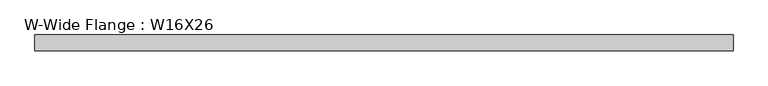
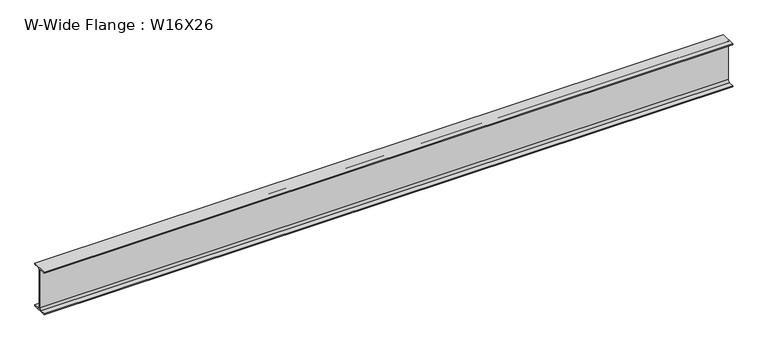
"""IFC4 building model written with IfcOpenShell, lengths in millimetres: beam geometry, W-Wide Flange : W16X26."""

from ifc_helpers import new_model, si_unit, point, frame, frame_2d, origin, place, context, project, spatial, polyline, circle_curve, trimmed, segment, composite_curve, outline, extrude, source, transform, mapped, element, save


def w_wide_flange_w16x26_1833ff5e(model_context):
    return source(origin(), model_context, "Body", "SweptSolid", [
        extrude(outline(composite_curve([segment(polyline([(69.85, -190.627), (69.85, -199.39), (-69.85, -199.39), (-69.85, -190.627), (-21.3995, -190.627)]), True, "CONTINUOUS"), segment(trimmed(circle_curve(frame_2d((-21.3995, -172.4025)), 18.2245), [point((-21.3995, -190.627))], [point((-3.175, -172.4025))], True, "CARTESIAN"), True, "CONTINUOUS"), segment(polyline([(-3.175, -172.4025), (-3.175, 172.4025)]), True, "CONTINUOUS"), segment(trimmed(circle_curve(frame_2d((-21.3995, 172.4025)), 18.2245), [point((-3.175, 172.4025))], [point((-21.3995, 190.627))], True, "CARTESIAN"), True, "CONTINUOUS"), segment(polyline([(-21.3995, 190.627), (-69.85, 190.627), (-69.85, 199.39), (69.85, 199.39), (69.85, 190.627), (21.3995, 190.627)]), True, "CONTINUOUS"), segment(trimmed(circle_curve(frame_2d((21.3995, 172.4025)), 18.2245), [point((21.3995, 190.627))], [point((3.175, 172.4025))], True, "CARTESIAN"), True, "CONTINUOUS"), segment(polyline([(3.175, 172.4025), (3.175, -172.4025)]), True, "CONTINUOUS"), segment(trimmed(circle_curve(frame_2d((21.3995, -172.4025)), 18.2245), [point((3.175, -172.4025))], [point((21.3995, -190.627))], True, "CARTESIAN"), True, "CONTINUOUS"), segment(polyline([(21.3995, -190.627), (69.85, -190.627)]), True, "CONTINUOUS")], self_intersect=False)), frame((-3048.0, 0.0, 0.0), z_axis=(1.0, 0.0, 0.0), x_axis=(0.0, 1.0, 0.0)), (0.0, 0.0, 1.0), 6096.0),
    ])


if __name__ == "__main__":
    model = new_model("IFC4")
    model_context = context("Model", 3, world=origin())
    ifc_project = project(units=[si_unit("LENGTHUNIT", "METRE", prefix="MILLI")], contexts=[model_context])
    site = spatial("IfcSite", under=ifc_project)
    building = spatial("IfcBuilding", under=site)
    placement = place(None, origin())
    w_wide_flange_w16x26_shape = w_wide_flange_w16x26_1833ff5e(model_context)
    element("IfcBeam", 1, ObjectType="W-Wide Flange : W16X26", at=placement, inside=building, context=model_context, shape_type="MappedRepresentation", body=[
        mapped(w_wide_flange_w16x26_shape, transform((0.0, 0.0, 0.0), x_axis=(1.0, 0.0, 0.0), y_axis=(0.0, 1.0, 0.0), z_axis=(0.0, 0.0, 1.0))),
    ])
    save(model, "model.ifc")

# Revit data of these elements
# Type "W-Wide Flange : W16X26"
#   Assembly Code = "B10"
#   W = 26
#   Length [instance default] = 5' - 0"
#   bf = 0' - 5 1/2"
#   d = 1' - 3.7"
#   k = 0' - 1 1/16"
#   k2 = 0' - 0.7175"
#   tf = 0' - 0.345"
#   tw = 0' - 0 1/4"
#   A = 0.0533333 SF
#   Structural Material [instance default] = Steel ASTM A992
# Element 1 (IfcBeam, "W-Wide Flange : W16X26")
#   Structural Material = Steel ASTM A36
#   Materials on its faces: "Steel ASTM A36"
# Materials
#   "Steel ASTM A992": class "Metal", colour RGB 199 199 199, transparency 0, Description = "Structural steel 50ksi", Cost = 0
#   "Steel ASTM A36": class "Metal", colour RGB 199 199 199, transparency 0, Description = "Structural steel, ASTM A36 Grade B, mill finish", Cost = 0
